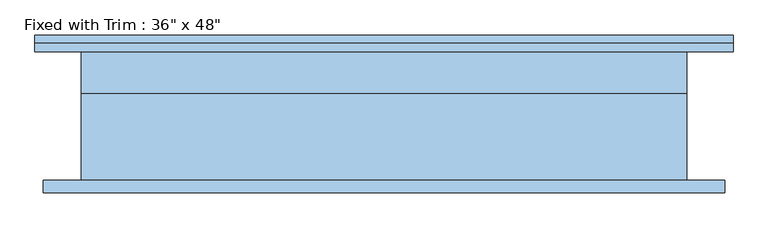
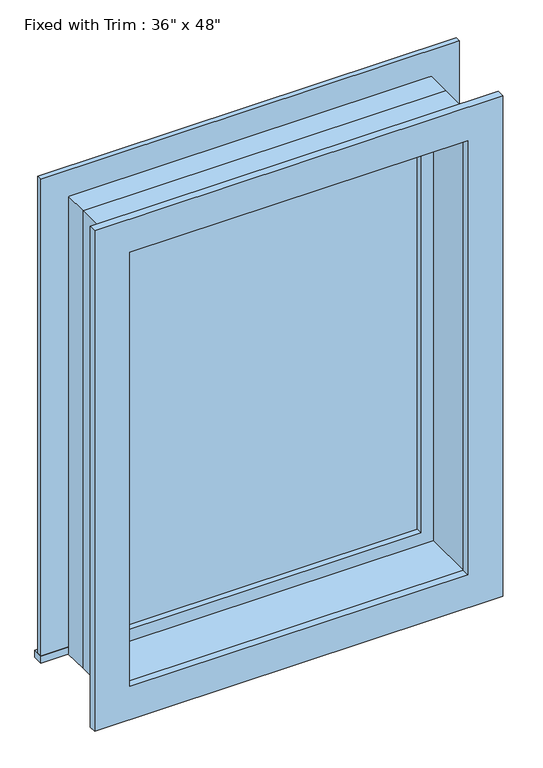
"""IFC4 building model written with IfcOpenShell, lengths in millimetres: window geometry."""

from ifc_helpers import new_model, si_unit, frame, origin, place, context, project, spatial, polyline, outline, extrude, source, transform, mapped, element, save


def window_31be35ed(model_context):
    return source(origin(), model_context, "Body", "SweptSolid", [
        extrude(outline(polyline([(-565.15, 122.2375), (488.95, 122.2375), (488.95, 96.8375), (-565.15, 96.8375), (-565.15, 122.2375)])), frame((0.0, 0.0, 914.4), z_axis=(0.0, 0.0, 1.0), x_axis=(1.0, 0.0, 0.0)), (0.0, 0.0, 1.0), 19.05),
        extrude(outline(polyline([(2114.55, -476.25), (2114.55, 400.05), (933.45, 400.05), (933.45, 488.95), (2203.45, 488.95), (2203.45, -565.15), (933.45, -565.15), (933.45, -476.25), (2114.55, -476.25)])), frame((0.0, 96.8375, 0.0), z_axis=(0.0, 1.0, 0.0), x_axis=(0.0, 0.0, 1.0)), (0.0, 0.0, 1.0), 12.7),
        extrude(outline(polyline([(2190.75, 476.25), (2190.75, -552.45), (857.25, -552.45), (857.25, 476.25), (2190.75, 476.25)]), holes=[polyline([(2101.85, 387.35), (946.15, 387.35), (946.15, -463.55), (2101.85, -463.55), (2101.85, 387.35)])]), frame((0.0, -115.8875, 0.0), z_axis=(0.0, 1.0, 0.0), x_axis=(0.0, 0.0, 1.0)), (0.0, 0.0, 1.0), 19.05),
        extrude(outline(polyline([(355.6, 49.2125), (-431.8, 49.2125), (-431.8, 61.9125), (355.6, 61.9125), (355.6, 49.2125)])), frame((0.0, 0.0, 977.9), z_axis=(0.0, 0.0, 1.0), x_axis=(1.0, 0.0, 0.0)), (0.0, 0.0, 1.0), 1092.2),
        extrude(outline(polyline([(2114.55, -476.25), (933.45, -476.25), (933.45, 400.05), (2114.55, 400.05), (2114.55, -476.25)]), holes=[polyline([(2070.1, -431.8), (2070.1, 355.6), (977.9, 355.6), (977.9, -431.8), (2070.1, -431.8)])]), frame((0.0, 33.3375, 0.0), z_axis=(0.0, 1.0, 0.0), x_axis=(0.0, 0.0, 1.0)), (0.0, 0.0, 1.0), 44.45),
        extrude(outline(polyline([(2133.6, -495.3), (914.4, -495.3), (914.4, 419.1), (2133.6, 419.1), (2133.6, -495.3)]), holes=[polyline([(2101.85, -463.55), (2101.85, 387.35), (946.15, 387.35), (946.15, -463.55), (2101.85, -463.55)])]), frame((0.0, -96.8375, 0.0), z_axis=(0.0, 1.0, 0.0), x_axis=(0.0, 0.0, 1.0)), (0.0, 0.0, 1.0), 130.175),
        extrude(outline(polyline([(2133.6, 419.1), (2133.6, -495.3), (914.4, -495.3), (914.4, 419.1), (2133.6, 419.1)]), holes=[polyline([(2114.55, 400.05), (933.45, 400.05), (933.45, -476.25), (2114.55, -476.25), (2114.55, 400.05)])]), frame((0.0, 33.3375, 0.0), z_axis=(0.0, 1.0, 0.0), x_axis=(0.0, 0.0, 1.0)), (0.0, 0.0, 1.0), 63.5),
    ])


if __name__ == "__main__":
    model = new_model("IFC4")
    model_context = context("Model", 3, world=origin())
    ifc_project = project(units=[si_unit("LENGTHUNIT", "METRE", prefix="MILLI")], contexts=[model_context])
    site = spatial("IfcSite", under=ifc_project)
    building = spatial("IfcBuilding", under=site)
    placement = place(None, origin())
    window_shape = window_31be35ed(model_context)
    element("IfcWindow", 1, ObjectType="Fixed with Trim : 36\" x 48\"", at=placement, inside=building, context=model_context, shape_type="MappedRepresentation", body=[
        mapped(window_shape, transform((0.0, 0.0, 0.0), x_axis=(1.0, 0.0, 0.0), y_axis=(0.0, 1.0, 0.0), z_axis=(0.0, 0.0, 1.0))),
    ])
    save(model, "model.ifc")

# Revit data of these elements
# Type "Fixed with Trim : 36\" x 48\""
#   Type Mark = "46"
#   Assembly Code = "B2020100"
#   Height = 4' - 0"
#   Default Sill Height = 3' - 0"
#   Trim Projection - Ext. = 0' - 0 1/2"
#   Trim Projection - Int. = 0' - 0 3/4"
#   Trim Width - Exterior = 0' - 3 1/2"
#   Trim Width - Interior = 0' - 3 1/2"
#   Width = 3' - 0"
#   Window Inset = 0' - 0 3/4"
#   Define Thermal Properties by = 0
#   Glass Pane Material = Glass
#   Sash Material = Sash
#   Trim Exterior Material = Trim
#   Trim Interior Material = Trim
#   Wall Closure = (empty or 0)
# Element 1 (IfcWindow, "Fixed with Trim : 36\" x 48\"")
#   Materials on its faces: "Sash", "Trim", "Glass"
# Materials
#   "Glass": class "Glass", colour RGB 236 240 239, transparency 0.5, Description = "Soda Lime Glass", Cost = 0
#   "Sash": class "Wood", colour RGB 227 170 128, transparency 0, Cost = 0
#   "Trim": class "Wood", colour RGB 227 170 128, transparency 0, Cost = 0
